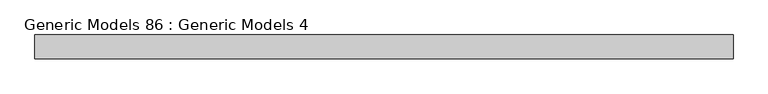
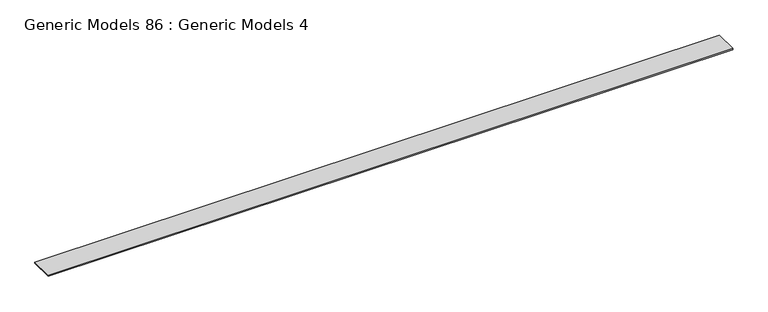
"""IFC4 building model written with IfcOpenShell, lengths in millimetres: proxy geometry, Generic Models 86 : Generic Models 4."""

import ifcopenshell
import ifcopenshell.guid

model = None  # the IFC model being written
_history = None  # IfcOwnerHistory: only IFC2X3 demands one
_inside = {}  # id of a spatial element -> (the spatial element, [elements in it])
_under = {}  # id of a project, library or spatial element -> (it, [spatial elements below it])
_declared = {}  # id of a project -> (the project, [libraries it declares])
_typed = {}  # id of a type object -> (the type object, [elements of that type])
_made_of = {}  # id of a material, layer set ... -> (it, [elements and type objects made of it])


def new_model(schema):
    """Start an empty IFC model of exactly this schema.

    Asked for "IFC4X3", IfcOpenShell would pick the latest addendum, in which some entities
    have other attributes; the version numbers below select the first issue.
    IFC2X3 requires an IfcOwnerHistory on every rooted entity: one is made here for all.
    """
    global model, _history
    if schema == "IFC4X3":
        model = ifcopenshell.file(schema_version=(4, 3, 0, 0))
    else:
        model = ifcopenshell.file(schema=schema)
    _inside.clear()
    _under.clear()
    _declared.clear()
    _typed.clear()
    _made_of.clear()
    _history = None
    if model.schema == "IFC2X3":
        org = make("IfcOrganization", Name="unknown")
        user = make(
            "IfcPersonAndOrganization",
            ThePerson=make("IfcPerson", FamilyName="unknown"),
            TheOrganization=org,
        )
        app = make(
            "IfcApplication",
            ApplicationDeveloper=org,
            Version="unknown",
            ApplicationFullName="unknown",
            ApplicationIdentifier="unknown",
        )
        _history = make(
            "IfcOwnerHistory",
            OwningUser=user,
            OwningApplication=app,
            ChangeAction="ADDED",
            CreationDate=0,
        )
    return model


def make(cls, **values):
    """One entity of the class cls with the attributes given. An attribute that is None is left unset."""
    return model.create_entity(
        cls, **{name: value for name, value in values.items() if value is not None}
    )


def rooted(cls, **values):
    """An entity with a GlobalId (a new one), such as an element, a storey or a relation."""
    return make(cls, GlobalId=ifcopenshell.guid.new(), OwnerHistory=_history, **values)


def si_unit(unit_type, name, prefix=None):
    """IfcSIUnit, for example si_unit("LENGTHUNIT", "METRE", prefix="MILLI")."""
    return make("IfcSIUnit", UnitType=unit_type, Prefix=prefix, Name=name)


def assignment(units):
    """IfcUnitAssignment: the units of a project."""
    return None if units is None else make("IfcUnitAssignment", Units=units)


def point(xyz):
    """IfcCartesianPoint."""
    return None if xyz is None else make("IfcCartesianPoint", Coordinates=xyz)


def direction(xyz):
    """IfcDirection."""
    return None if xyz is None else make("IfcDirection", DirectionRatios=xyz)


def frame(location, z_axis=None, x_axis=None):
    """IfcAxis2Placement3D, a coordinate frame: its origin and axes. An axis left out is left unset."""
    return make(
        "IfcAxis2Placement3D",
        Location=point(location),
        Axis=direction(z_axis),
        RefDirection=direction(x_axis),
    )


def origin():
    """The frame at (0, 0, 0) with its axes left unset."""
    return frame((0.0, 0.0, 0.0))


def place(relative_to, where):
    """IfcLocalPlacement: puts the frame where relative to a parent placement (None: the world)."""
    return make(
        "IfcLocalPlacement", PlacementRelTo=relative_to, RelativePlacement=where
    )


def context(
    kind, dimensions, precision=None, world=None, true_north=None, identifier=None
):
    """IfcGeometricRepresentationContext, for example the 3D "Model" context."""
    return make(
        "IfcGeometricRepresentationContext",
        ContextIdentifier=identifier,
        ContextType=kind,
        CoordinateSpaceDimension=dimensions,
        Precision=precision,
        WorldCoordinateSystem=world,
        TrueNorth=true_north,
    )


def project(units=None, contexts=None):
    """IfcProject with its units and contexts."""
    return rooted(
        "IfcProject",
        Name="project",
        RepresentationContexts=contexts,
        UnitsInContext=assignment(units),
    )


def spatial(cls, under=None, at=None, **own):
    """A site, building, storey or space (cls), placed at a placement, below another one or the project."""
    s = rooted(cls, ObjectPlacement=at, **own)
    if under is not None:
        _under.setdefault(under.id(), (under, []))[1].append(s)
    return s


def polyline(points):
    """IfcPolyline through the points."""
    return make("IfcPolyline", Points=[point(p) for p in points])


def outline(outer, holes=None, kind="AREA"):
    """IfcArbitraryClosedProfileDef: a profile drawn as a closed curve; with holes, ...WithVoids."""
    if holes is None:
        return make("IfcArbitraryClosedProfileDef", ProfileType=kind, OuterCurve=outer)
    return make(
        "IfcArbitraryProfileDefWithVoids",
        ProfileType=kind,
        OuterCurve=outer,
        InnerCurves=holes,
    )


def extrude(swept, where, along, depth):
    """IfcExtrudedAreaSolid: the profile swept, set in the frame where, extruded along a direction by depth."""
    return make(
        "IfcExtrudedAreaSolid",
        SweptArea=swept,
        Position=where,
        ExtrudedDirection=direction(along),
        Depth=depth,
    )


def shape(context_of_items, identifier, shape_type, items):
    """IfcShapeRepresentation: the items that make up one representation, for example the "Body"."""
    return make(
        "IfcShapeRepresentation",
        ContextOfItems=context_of_items,
        RepresentationIdentifier=identifier,
        RepresentationType=shape_type,
        Items=items,
    )


def source(mapping_origin, context_of_items, identifier, shape_type, items):
    """IfcRepresentationMap: a shape defined once, which mapped items show again and again."""
    return make(
        "IfcRepresentationMap",
        MappingOrigin=mapping_origin,
        MappedRepresentation=shape(context_of_items, identifier, shape_type, items),
    )


def transform(
    local_origin,
    x_axis=None,
    y_axis=None,
    z_axis=None,
    scale=None,
    scale2=None,
    scale3=None,
    uniform=True,
):
    """IfcCartesianTransformationOperator3D, or its non-uniform kind. x_axis, y_axis, z_axis: its Axis1, 2, 3."""
    if uniform:
        return make(
            "IfcCartesianTransformationOperator3D",
            Axis1=direction(x_axis),
            Axis2=direction(y_axis),
            LocalOrigin=point(local_origin),
            Scale=scale,
            Axis3=direction(z_axis),
        )
    return make(
        "IfcCartesianTransformationOperator3DnonUniform",
        Axis1=direction(x_axis),
        Axis2=direction(y_axis),
        LocalOrigin=point(local_origin),
        Scale=scale,
        Axis3=direction(z_axis),
        Scale2=scale2,
        Scale3=scale3,
    )


def mapped(mapping_source, mapping_target):
    """IfcMappedItem: shows the shape of a source again, moved by a transform."""
    return make(
        "IfcMappedItem", MappingSource=mapping_source, MappingTarget=mapping_target
    )


def made_of(thing, what):
    """Note that an element or type object is made of a material, layer set ...; save() writes the relation."""
    if what is not None:
        _made_of.setdefault(what.id(), (what, []))[1].append(thing)
    return thing


def element(
    cls,
    number,
    at=None,
    inside=None,
    cuts=None,
    type_object=None,
    material=None,
    context=None,
    identifier="Body",
    shape_type=None,
    held_by="IfcProductDefinitionShape",
    body=None,
    shapes=None,
    **own,
):
    """One element of the class cls, such as IfcWall. Its Tag is "e" and its number.

    at: its placement. inside: the storey or other place that contains it. cuts: it is an
    opening in that element (IfcRelVoidsElement). A single representation is given by context,
    identifier, shape_type and body (its items); several are given by shapes. held_by: the class
    of the entity that holds the representations. save() writes the other relations.
    """
    e = rooted(cls, Tag="e%d" % number, ObjectPlacement=at, **own)
    if body is not None:
        shapes = [shape(context, identifier, shape_type, body)]
    if shapes is not None:
        e.Representation = make(held_by, Representations=shapes)
    if inside is not None:
        _inside.setdefault(inside.id(), (inside, []))[1].append(e)
    if cuts is not None:
        rooted(
            "IfcRelVoidsElement", RelatingBuildingElement=cuts, RelatedOpeningElement=e
        )
    if type_object is not None:
        _typed.setdefault(type_object.id(), (type_object, []))[1].append(e)
    return made_of(e, material)


def aggregate(whole, parts):
    """IfcRelAggregates: a whole, such as a stair, and the parts it consists of."""
    return rooted("IfcRelAggregates", RelatingObject=whole, RelatedObjects=parts)


def save(model, path):
    """Write the relations noted so far, then the file.

    IfcRelAggregates (storeys below a building ...), IfcRelContainedInSpatialStructure (elements
    in a storey), IfcRelDefinesByType, IfcRelAssociatesMaterial and IfcRelDeclares: one each for
    every whole, place, type object, material and project.
    """
    for whole, parts in _under.values():
        aggregate(whole, parts)
    for where, things in _inside.values():
        rooted(
            "IfcRelContainedInSpatialStructure",
            RelatedElements=things,
            RelatingStructure=where,
        )
    for kind, things in _typed.values():
        rooted("IfcRelDefinesByType", RelatedObjects=things, RelatingType=kind)
    for what, things in _made_of.values():
        rooted("IfcRelAssociatesMaterial", RelatedObjects=things, RelatingMaterial=what)
    for by, libraries in _declared.values():
        rooted("IfcRelDeclares", RelatingContext=by, RelatedDefinitions=libraries)
    model.write(path)


def generic_models_86_generic_models_4_2027ced3(model_context):
    return source(origin(), model_context, "Body", "SweptSolid", [
        extrude(outline(polyline([(0.0, -211.2582119), (0.0, 0.0), (6219.2994598, 0.0), (6219.2994598, -211.2582119), (0.0, -211.2582119)])), frame((-2152.1733045, 16455.0628894, 126343.2450925), z_axis=(0.0, 0.02082881368192768, 0.9997830567281102), x_axis=(-1.0, 0.0, 0.0)), (0.0, 0.0, 1.0), 12.7),
    ])


if __name__ == "__main__":
    model = new_model("IFC4")
    model_context = context("Model", 3, world=origin())
    ifc_project = project(units=[si_unit("LENGTHUNIT", "METRE", prefix="MILLI")], contexts=[model_context])
    site = spatial("IfcSite", under=ifc_project)
    building = spatial("IfcBuilding", under=site)
    placement = place(None, origin())
    generic_models_86_generic_models_4_shape = generic_models_86_generic_models_4_2027ced3(model_context)
    element("IfcBuildingElementProxy", 1, Name="Generic Models 86 : Generic Models 4", ObjectType="Generic Models 86 : Generic Models 4", at=placement, inside=building, context=model_context, shape_type="MappedRepresentation", body=[
        mapped(generic_models_86_generic_models_4_shape, transform((0.0, 0.0, 0.0), x_axis=(1.0, 0.0, 0.0), y_axis=(0.0, 1.0, 0.0), z_axis=(0.0, 0.0, 1.0))),
    ])
    save(model, "model.ifc")

# Revit data of these elements
# Element 1 (IfcBuildingElementProxy, "Generic Models 86 : Generic Models 4")
#   Materials on its faces: "_1/2\" CDX PLYWOOD"
# Materials
#   "_1/2\" CDX PLYWOOD": class "Generic", colour RGB 98 75 74, transparency 0, Cost = 0
